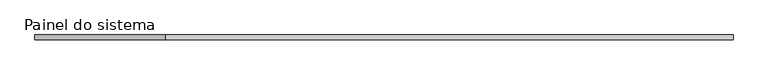
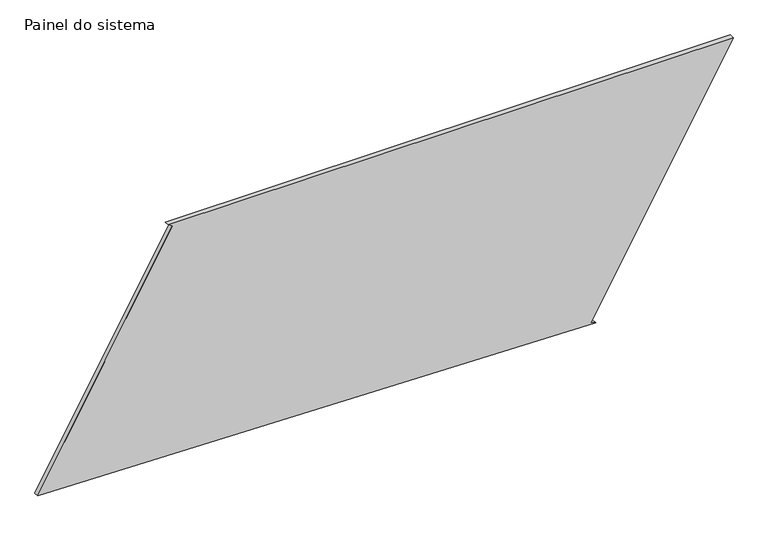
"""IFC4 building model written with IfcOpenShell, lengths in millimetres: plate geometry, Painel do sistema : Envidraçado."""

from ifc_helpers import new_model, si_unit, frame, origin, place, context, project, spatial, polyline, outline, extrude, source, transform, mapped, element, save


def painel_do_sistema_200ed0e2(model_context):
    return source(origin(), model_context, "Body", "SweptSolid", [
        extrude(outline(polyline([(0.0, 1088.733569), (12.2820845, 1066.9585742), (1311.9833643, 1800.0490361), (1311.9833643, -1124.8987767), (1299.7012798, -1103.1237818), (64.1175532, -1800.0490361), (0.0, 1088.733569)])), frame((0.0, 24.5, 0.0), z_axis=(0.0, 1.0, 0.0), x_axis=(0.0, 0.0, 1.0)), (0.0, 0.0, 1.0), 25.0),
    ])


if __name__ == "__main__":
    model = new_model("IFC4")
    model_context = context("Model", 3, world=origin())
    ifc_project = project(units=[si_unit("LENGTHUNIT", "METRE", prefix="MILLI")], contexts=[model_context])
    site = spatial("IfcSite", under=ifc_project)
    building = spatial("IfcBuilding", under=site)
    placement = place(None, origin())
    painel_do_sistema_shape = painel_do_sistema_200ed0e2(model_context)
    element("IfcPlate", 1, ObjectType="Painel do sistema : Envidraçado", at=placement, inside=building, context=model_context, shape_type="MappedRepresentation", body=[
        mapped(painel_do_sistema_shape, transform((0.0, 0.0, 0.0), x_axis=(1.0, 0.0, 0.0), y_axis=(0.0, 1.0, 0.0), z_axis=(0.0, 0.0, 1.0))),
    ])
    save(model, "model.ifc")

# Revit data of these elements
# Type "Painel do sistema : Envidraçado"
#   Construction Type Id = "GSP4R"
#   Analytic Construction = "Vidraça única Pilkington 1/8 pol"
#   Visual Light Transmittance = 0.9
#   Solar Heat Gain Coefficient = 0.86
#   Heat Transfer Coefficient (U) = 6.7069 W/(m²·K)
# Element 1 (IfcPlate, "Painel do sistema : Envidraçado")
#   Materials on its faces: "Vidro"
# Materials
#   "Vidro": class "Vidro", colour RGB 0 128 192, transparency 0.9, Description = "Vidro de sílica", Cost = 0
